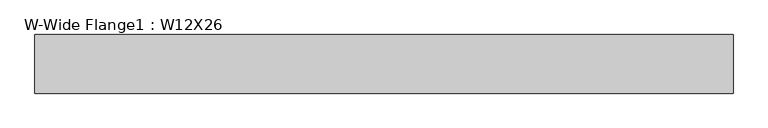
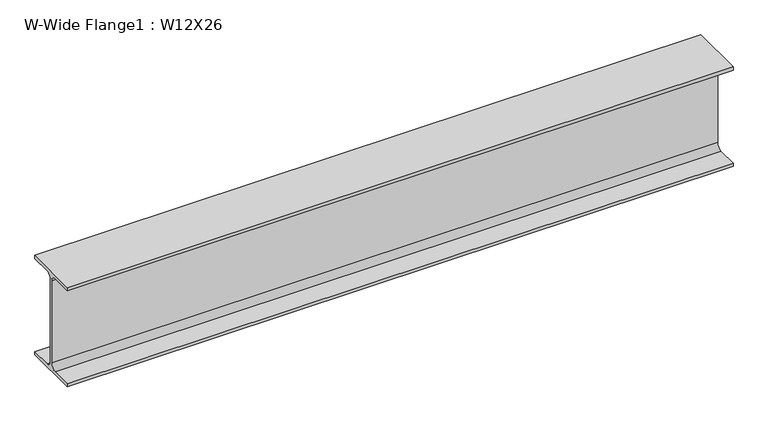
"""IFC4 building model written with IfcOpenShell, lengths in millimetres: beam geometry, W-Wide Flange1 : W12X26."""

from ifc_helpers import new_model, si_unit, point, frame, frame_2d, origin, place, context, project, spatial, polyline, circle_curve, trimmed, segment, composite_curve, outline, extrude, source, transform, mapped, element, save


def w_wide_flange1_w12x26_c48f6713(model_context):
    return source(origin(), model_context, "Body", "SweptSolid", [
        extrude(outline(composite_curve([segment(polyline([(82.423, -145.288), (82.423, -154.94), (-82.423, -154.94), (-82.423, -145.288), (-20.2565, -145.288)]), True, "CONTINUOUS"), segment(trimmed(circle_curve(frame_2d((-20.2565, -127.9525)), 17.3355), [point((-20.2565, -145.288))], [point((-2.921, -127.9525))], True, "CARTESIAN"), True, "CONTINUOUS"), segment(polyline([(-2.921, -127.9525), (-2.921, 127.9525)]), True, "CONTINUOUS"), segment(trimmed(circle_curve(frame_2d((-20.2565, 127.9525)), 17.3355), [point((-2.921, 127.9525))], [point((-20.2565, 145.288))], True, "CARTESIAN"), True, "CONTINUOUS"), segment(polyline([(-20.2565, 145.288), (-82.423, 145.288), (-82.423, 154.94), (82.423, 154.94), (82.423, 145.288), (20.2565, 145.288)]), True, "CONTINUOUS"), segment(trimmed(circle_curve(frame_2d((20.2565, 127.9525)), 17.3355), [point((20.2565, 145.288))], [point((2.921, 127.9525))], True, "CARTESIAN"), True, "CONTINUOUS"), segment(polyline([(2.921, 127.9525), (2.921, -127.9525)]), True, "CONTINUOUS"), segment(trimmed(circle_curve(frame_2d((20.2565, -127.9525)), 17.3355), [point((2.921, -127.9525))], [point((20.2565, -145.288))], True, "CARTESIAN"), True, "CONTINUOUS"), segment(polyline([(20.2565, -145.288), (82.423, -145.288)]), True, "CONTINUOUS")], self_intersect=False)), frame((-876.7347683, 0.0, 0.0), z_axis=(1.0, 0.0, 0.0), x_axis=(0.0, 1.0, 0.0)), (0.0, 0.0, 1.0), 1962.6844888),
    ])


if __name__ == "__main__":
    model = new_model("IFC4")
    model_context = context("Model", 3, world=origin())
    ifc_project = project(units=[si_unit("LENGTHUNIT", "METRE", prefix="MILLI")], contexts=[model_context])
    site = spatial("IfcSite", under=ifc_project)
    building = spatial("IfcBuilding", under=site)
    placement = place(None, origin())
    w_wide_flange1_w12x26_shape = w_wide_flange1_w12x26_c48f6713(model_context)
    element("IfcBeam", 1, ObjectType="W-Wide Flange1 : W12X26", at=placement, inside=building, context=model_context, shape_type="MappedRepresentation", body=[
        mapped(w_wide_flange1_w12x26_shape, transform((0.0, 0.0, 0.0), x_axis=(1.0, 0.0, 0.0), y_axis=(0.0, 1.0, 0.0), z_axis=(0.0, 0.0, 1.0))),
    ])
    save(model, "model.ifc")

# Revit data of these elements
# Type "W-Wide Flange1 : W12X26"
#   Assembly Code = "B10"
#   W = 26
#   Start Extension Calculation [instance default] = 10' - 0"
#   Start Extension [instance default] = -0' - 0 1/2"
#   End Extension Calculation [instance default] = 10' - 0"
#   End Extension [instance default] = -0' - 0 1/2"
#   Length [instance default] = 5' - 0"
#   bf = 0' - 6.49"
#   d = 1' - 0.2"
#   k = 0' - 1 1/16"
#   k2 = 0' - 0.6825"
#   tf = 0' - 0.38"
#   tw = 0' - 0.23"
#   A = 0.053125 SF
#   Structural Material [instance default] = Metal - Steel - ASTM A992
# Element 1 (IfcBeam, "W-Wide Flange1 : W12X26")
#   Materials on its faces: "Metal - Steel - ASTM A992"
# Materials
#   "Metal - Steel - ASTM A992": class "Metal", colour RGB 199 199 199, transparency 0
